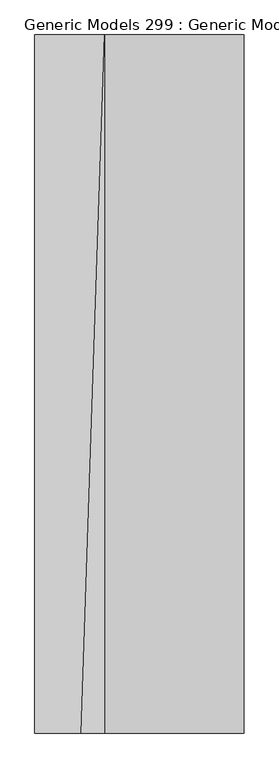
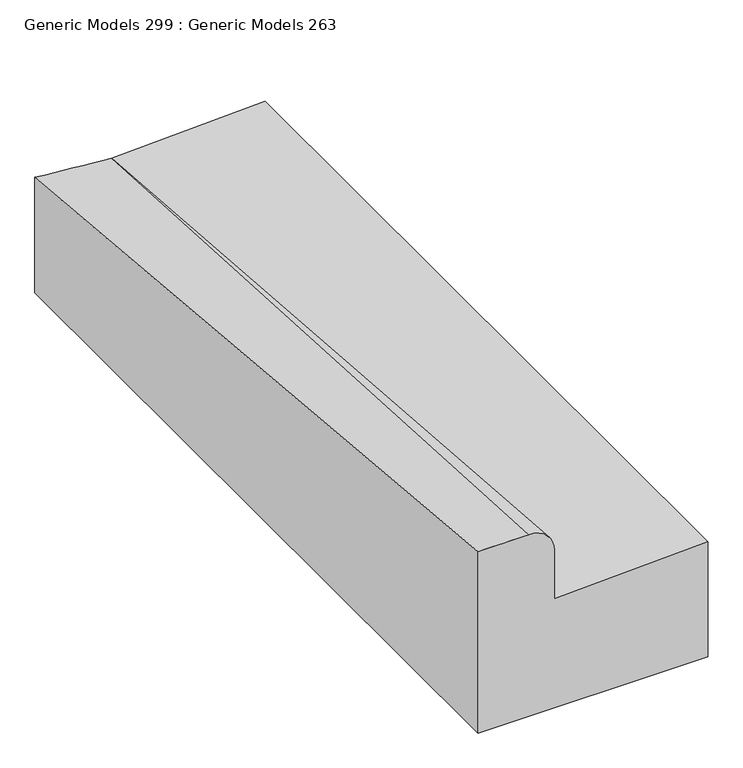
"""IFC4 building model written with IfcOpenShell, lengths in millimetres: proxy geometry, Generic Models 299 : Generic Models 263."""

import ifcopenshell
import ifcopenshell.guid

model = None  # the IFC model being written
_history = None  # IfcOwnerHistory: only IFC2X3 demands one
_inside = {}  # id of a spatial element -> (the spatial element, [elements in it])
_under = {}  # id of a project, library or spatial element -> (it, [spatial elements below it])
_declared = {}  # id of a project -> (the project, [libraries it declares])
_typed = {}  # id of a type object -> (the type object, [elements of that type])
_made_of = {}  # id of a material, layer set ... -> (it, [elements and type objects made of it])


def new_model(schema):
    """Start an empty IFC model of exactly this schema.

    Asked for "IFC4X3", IfcOpenShell would pick the latest addendum, in which some entities
    have other attributes; the version numbers below select the first issue.
    IFC2X3 requires an IfcOwnerHistory on every rooted entity: one is made here for all.
    """
    global model, _history
    if schema == "IFC4X3":
        model = ifcopenshell.file(schema_version=(4, 3, 0, 0))
    else:
        model = ifcopenshell.file(schema=schema)
    _inside.clear()
    _under.clear()
    _declared.clear()
    _typed.clear()
    _made_of.clear()
    _history = None
    if model.schema == "IFC2X3":
        org = make("IfcOrganization", Name="unknown")
        user = make(
            "IfcPersonAndOrganization",
            ThePerson=make("IfcPerson", FamilyName="unknown"),
            TheOrganization=org,
        )
        app = make(
            "IfcApplication",
            ApplicationDeveloper=org,
            Version="unknown",
            ApplicationFullName="unknown",
            ApplicationIdentifier="unknown",
        )
        _history = make(
            "IfcOwnerHistory",
            OwningUser=user,
            OwningApplication=app,
            ChangeAction="ADDED",
            CreationDate=0,
        )
    return model


def make(cls, **values):
    """One entity of the class cls with the attributes given. An attribute that is None is left unset."""
    return model.create_entity(
        cls, **{name: value for name, value in values.items() if value is not None}
    )


def rooted(cls, **values):
    """An entity with a GlobalId (a new one), such as an element, a storey or a relation."""
    return make(cls, GlobalId=ifcopenshell.guid.new(), OwnerHistory=_history, **values)


def si_unit(unit_type, name, prefix=None):
    """IfcSIUnit, for example si_unit("LENGTHUNIT", "METRE", prefix="MILLI")."""
    return make("IfcSIUnit", UnitType=unit_type, Prefix=prefix, Name=name)


def assignment(units):
    """IfcUnitAssignment: the units of a project."""
    return None if units is None else make("IfcUnitAssignment", Units=units)


def point(xyz):
    """IfcCartesianPoint."""
    return None if xyz is None else make("IfcCartesianPoint", Coordinates=xyz)


def direction(xyz):
    """IfcDirection."""
    return None if xyz is None else make("IfcDirection", DirectionRatios=xyz)


def frame(location, z_axis=None, x_axis=None):
    """IfcAxis2Placement3D, a coordinate frame: its origin and axes. An axis left out is left unset."""
    return make(
        "IfcAxis2Placement3D",
        Location=point(location),
        Axis=direction(z_axis),
        RefDirection=direction(x_axis),
    )


def origin():
    """The frame at (0, 0, 0) with its axes left unset."""
    return frame((0.0, 0.0, 0.0))


def place(relative_to, where):
    """IfcLocalPlacement: puts the frame where relative to a parent placement (None: the world)."""
    return make(
        "IfcLocalPlacement", PlacementRelTo=relative_to, RelativePlacement=where
    )


def context(
    kind, dimensions, precision=None, world=None, true_north=None, identifier=None
):
    """IfcGeometricRepresentationContext, for example the 3D "Model" context."""
    return make(
        "IfcGeometricRepresentationContext",
        ContextIdentifier=identifier,
        ContextType=kind,
        CoordinateSpaceDimension=dimensions,
        Precision=precision,
        WorldCoordinateSystem=world,
        TrueNorth=true_north,
    )


def project(units=None, contexts=None):
    """IfcProject with its units and contexts."""
    return rooted(
        "IfcProject",
        Name="project",
        RepresentationContexts=contexts,
        UnitsInContext=assignment(units),
    )


def spatial(cls, under=None, at=None, **own):
    """A site, building, storey or space (cls), placed at a placement, below another one or the project."""
    s = rooted(cls, ObjectPlacement=at, **own)
    if under is not None:
        _under.setdefault(under.id(), (under, []))[1].append(s)
    return s


def circle_curve(where, radius):
    """IfcCircle in the frame where."""
    return make("IfcCircle", Position=where, Radius=radius)


def shape(context_of_items, identifier, shape_type, items):
    """IfcShapeRepresentation: the items that make up one representation, for example the "Body"."""
    return make(
        "IfcShapeRepresentation",
        ContextOfItems=context_of_items,
        RepresentationIdentifier=identifier,
        RepresentationType=shape_type,
        Items=items,
    )


def source(mapping_origin, context_of_items, identifier, shape_type, items):
    """IfcRepresentationMap: a shape defined once, which mapped items show again and again."""
    return make(
        "IfcRepresentationMap",
        MappingOrigin=mapping_origin,
        MappedRepresentation=shape(context_of_items, identifier, shape_type, items),
    )


def transform(
    local_origin,
    x_axis=None,
    y_axis=None,
    z_axis=None,
    scale=None,
    scale2=None,
    scale3=None,
    uniform=True,
):
    """IfcCartesianTransformationOperator3D, or its non-uniform kind. x_axis, y_axis, z_axis: its Axis1, 2, 3."""
    if uniform:
        return make(
            "IfcCartesianTransformationOperator3D",
            Axis1=direction(x_axis),
            Axis2=direction(y_axis),
            LocalOrigin=point(local_origin),
            Scale=scale,
            Axis3=direction(z_axis),
        )
    return make(
        "IfcCartesianTransformationOperator3DnonUniform",
        Axis1=direction(x_axis),
        Axis2=direction(y_axis),
        LocalOrigin=point(local_origin),
        Scale=scale,
        Axis3=direction(z_axis),
        Scale2=scale2,
        Scale3=scale3,
    )


def mapped(mapping_source, mapping_target):
    """IfcMappedItem: shows the shape of a source again, moved by a transform."""
    return make(
        "IfcMappedItem", MappingSource=mapping_source, MappingTarget=mapping_target
    )


def made_of(thing, what):
    """Note that an element or type object is made of a material, layer set ...; save() writes the relation."""
    if what is not None:
        _made_of.setdefault(what.id(), (what, []))[1].append(thing)
    return thing


def element(
    cls,
    number,
    at=None,
    inside=None,
    cuts=None,
    type_object=None,
    material=None,
    context=None,
    identifier="Body",
    shape_type=None,
    held_by="IfcProductDefinitionShape",
    body=None,
    shapes=None,
    **own,
):
    """One element of the class cls, such as IfcWall. Its Tag is "e" and its number.

    at: its placement. inside: the storey or other place that contains it. cuts: it is an
    opening in that element (IfcRelVoidsElement). A single representation is given by context,
    identifier, shape_type and body (its items); several are given by shapes. held_by: the class
    of the entity that holds the representations. save() writes the other relations.
    """
    e = rooted(cls, Tag="e%d" % number, ObjectPlacement=at, **own)
    if body is not None:
        shapes = [shape(context, identifier, shape_type, body)]
    if shapes is not None:
        e.Representation = make(held_by, Representations=shapes)
    if inside is not None:
        _inside.setdefault(inside.id(), (inside, []))[1].append(e)
    if cuts is not None:
        rooted(
            "IfcRelVoidsElement", RelatingBuildingElement=cuts, RelatedOpeningElement=e
        )
    if type_object is not None:
        _typed.setdefault(type_object.id(), (type_object, []))[1].append(e)
    return made_of(e, material)


def aggregate(whole, parts):
    """IfcRelAggregates: a whole, such as a stair, and the parts it consists of."""
    return rooted("IfcRelAggregates", RelatingObject=whole, RelatedObjects=parts)


def save(model, path):
    """Write the relations noted so far, then the file.

    IfcRelAggregates (storeys below a building ...), IfcRelContainedInSpatialStructure (elements
    in a storey), IfcRelDefinesByType, IfcRelAssociatesMaterial and IfcRelDeclares: one each for
    every whole, place, type object, material and project.
    """
    for whole, parts in _under.values():
        aggregate(whole, parts)
    for where, things in _inside.values():
        rooted(
            "IfcRelContainedInSpatialStructure",
            RelatedElements=things,
            RelatingStructure=where,
        )
    for kind, things in _typed.values():
        rooted("IfcRelDefinesByType", RelatedObjects=things, RelatingType=kind)
    for what, things in _made_of.values():
        rooted("IfcRelAssociatesMaterial", RelatedObjects=things, RelatingMaterial=what)
    for by, libraries in _declared.values():
        rooted("IfcRelDeclares", RelatingContext=by, RelatedDefinitions=libraries)
    model.write(path)


def plane_surface(at):
    """IfcPlane: the flat surface through the origin of the frame at, square to its z axis."""
    return make("IfcPlane", Position=at)


def spline_surface(u_degree, v_degree, points, u_multiplicities, v_multiplicities, u_knots, v_knots, weights=None):
    """IfcBSplineSurfaceWithKnots; with weights, IfcRationalBSplineSurfaceWithKnots. points: one row for each step in u."""
    own = dict(
        UDegree=u_degree,
        VDegree=v_degree,
        ControlPointsList=[[point(p) for p in row] for row in points],
        SurfaceForm="UNSPECIFIED",
        UClosed=False,
        VClosed=False,
        SelfIntersect=False,
        UMultiplicities=u_multiplicities,
        VMultiplicities=v_multiplicities,
        UKnots=u_knots,
        VKnots=v_knots,
        KnotSpec="UNSPECIFIED",
    )
    if weights is None:
        return make("IfcBSplineSurfaceWithKnots", **own)
    return make("IfcRationalBSplineSurfaceWithKnots", WeightsData=weights, **own)


def advanced_brep(points, edges, surfaces, faces):
    """IfcAdvancedBrep: a solid bounded by faces that lie on surfaces and meet in shared edges.

    An edge is (start, end): straight between two places in points (the first is 0);
    or (start, end, curve); or (start, end, curve, False) where it runs against its curve.
    A face is (place in surfaces, loops), or (place, loops, False) where it looks against
    its surface's normal. A loop lists edges by number (the first is 1), with a minus sign
    where the edge is run from its end to its start. The first loop is the outer one.
    """
    corners = [point(p) for p in points]
    vertices = [make("IfcVertexPoint", VertexGeometry=c) for c in corners]
    made = []
    for start, end, *more in edges:
        made.append(
            make(
                "IfcEdgeCurve",
                EdgeStart=vertices[start],
                EdgeEnd=vertices[end],
                EdgeGeometry=more[0] if more else make("IfcPolyline", Points=[corners[start], corners[end]]),
                SameSense=more[1] if len(more) > 1 else True,
            )
        )
    hull = []
    for where, loops, *sense in faces:
        bounds = []
        for j, loop in enumerate(loops):
            ring = [make("IfcOrientedEdge", EdgeElement=made[abs(k) - 1], Orientation=k > 0) for k in loop]
            bounds.append(
                make(
                    "IfcFaceOuterBound" if j == 0 else "IfcFaceBound",
                    Bound=make("IfcEdgeLoop", EdgeList=ring),
                    Orientation=True,
                )
            )
        hull.append(make("IfcAdvancedFace", Bounds=bounds, FaceSurface=surfaces[where], SameSense=sense[0] if sense else True))
    return make("IfcAdvancedBrep", Outer=make("IfcClosedShell", CfsFaces=hull))


def generic_models_299_generic_models_263_ab59c33a(model_context):
    return source(origin(), model_context, "Body", "AdvancedBrep", [
        advanced_brep(
        [(91579.9797726, -6732.6272578, -139.1379392), (91732.3797726, -6732.6272578, -152.4), (92037.1797726, -6732.6272578, -139.7), (92037.1797726, -6732.6272578, -381.0), (91579.9797726, -6732.6272578, -381.0), (91579.9797726, -8256.6272578, 0.0), (91579.9797726, -8256.6272578, -381.0), (92037.1797726, -8256.6272578, -381.0), (92037.1797726, -8256.6272578, -139.7), (91732.3797726, -8256.6272578, -152.4), (91732.3797726, -8256.6272578, -50.8), (91681.5797726, -8256.6272578, 0.0)],
        [
            (0, 1),
            (1, 2),
            (2, 3),
            (3, 4),
            (4, 0),
            (5, 6),
            (6, 7),
            (7, 8),
            (8, 9),
            (9, 10),
            (10, 11, circle_curve(frame((91681.5797726, -8256.6272578, -50.8), z_axis=(0.0, -1.0, 0.0), x_axis=(1.0, 0.0, 0.0)), 50.8)),
            (11, 5),
            (5, 0),
            (4, 6),
            (3, 7),
            (2, 8),
            (9, 1),
            (1, 10),
            (1, 11),
        ],
        [
            plane_surface(frame((91793.3397726, -6732.6272578, -238.6475878), z_axis=(0.0, 1.0, 0.0), x_axis=(0.0, 0.0, 1.0))),
            plane_surface(frame((91768.6654869, -8256.6272578, -157.8428571), z_axis=(0.0, -1.0, 0.0), x_axis=(0.0, 0.0, 1.0))),
            plane_surface(frame((91579.9797726, -8256.6272578, -190.5), z_axis=(-1.0, 0.0, 0.0), x_axis=(0.0, 0.0, 1.0))),
            plane_surface(frame((91808.5797726, -8256.6272578, -381.0), z_axis=(0.0, 0.0, -1.0), x_axis=(-1.0, 0.0, 0.0))),
            plane_surface(frame((92037.1797726, -8256.6272578, -260.35), z_axis=(1.0, 0.0, 0.0), x_axis=(0.0, 0.0, -1.0))),
            plane_surface(frame((91732.3797726, -8256.6272578, -101.6), z_axis=(1.0, 0.0, 0.0), x_axis=(0.0, 0.0, -1.0))),
            spline_surface(2, 1, [[(91681.5797726, -8256.6272578, 0.0), (91732.3797726, -6732.6272578, -152.4)], [(91732.3797726, -8256.6272578, -2.9132252166164108e-12), (91732.3797726, -6732.6272578, -152.4)], [(91732.3797726, -8256.6272578, -50.8), (91732.3797726, -6732.6272578, -152.4)]], [3, 3], [2, 2], [0.0, 1.0], [0.0, 1.0], weights=[[1.0, 1.0], [0.7071067811865678, 0.7071067811865678], [1.0, 1.0]]),
            spline_surface(1, 1, [[(91579.9797726, -8256.6272578, 0.0), (91579.9797726, -6732.6272578, -139.1379392)], [(91681.5797726, -8256.6272578, 0.0), (91732.3797726, -6732.6272578, -152.4)]], [2, 2], [2, 2], [0.0, 1.0], [0.0, 1.0]),
            plane_surface(frame((91884.7797726, -8256.6272578, -146.05), z_axis=(-0.04163054471218606, 0.0, 0.9991330730923518), x_axis=(0.9991330730923518, 0.0, 0.04163054471218606))),
        ],
        [
            (0, [[1, 2, 3, 4, 5]]),
            (1, [[6, 7, 8, 9, 10, 11, 12]]),
            (2, [[-6, 13, -5, 14]]),
            (3, [[-7, -14, -4, 15]]),
            (4, [[-8, -15, -3, 16]]),
            (5, [[-10, 17, 18]]),
            (6, [[-11, -18, 19]]),
            (7, [[-12, -19, -1, -13]]),
            (8, [[-9, -16, -2, -17]]),
        ],
    ),
    ])


if __name__ == "__main__":
    model = new_model("IFC4")
    model_context = context("Model", 3, world=origin())
    ifc_project = project(units=[si_unit("LENGTHUNIT", "METRE", prefix="MILLI")], contexts=[model_context])
    site = spatial("IfcSite", under=ifc_project)
    building = spatial("IfcBuilding", under=site)
    placement = place(None, origin())
    generic_models_299_generic_models_263_shape = generic_models_299_generic_models_263_ab59c33a(model_context)
    element("IfcBuildingElementProxy", 1, Name="Generic Models 299 : Generic Models 263", ObjectType="Generic Models 299 : Generic Models 263", at=placement, inside=building, context=model_context, shape_type="MappedRepresentation", body=[
        mapped(generic_models_299_generic_models_263_shape, transform((0.0, 0.0, 0.0), x_axis=(1.0, 0.0, 0.0), y_axis=(0.0, 1.0, 0.0), z_axis=(0.0, 0.0, 1.0))),
    ])
    save(model, "model.ifc")

# Revit data of these elements
# Element 1 (IfcBuildingElementProxy, "Generic Models 299 : Generic Models 263")
#   Materials on its faces: "CONCRETE CURB"
# Materials
#   "CONCRETE CURB": class "Concrete", colour RGB 191 191 191, transparency 0, Description = "Cast-in-place concrete", Cost = 0
